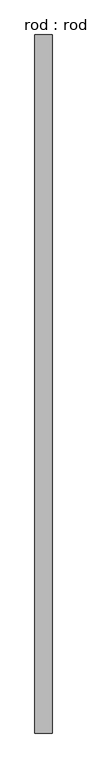
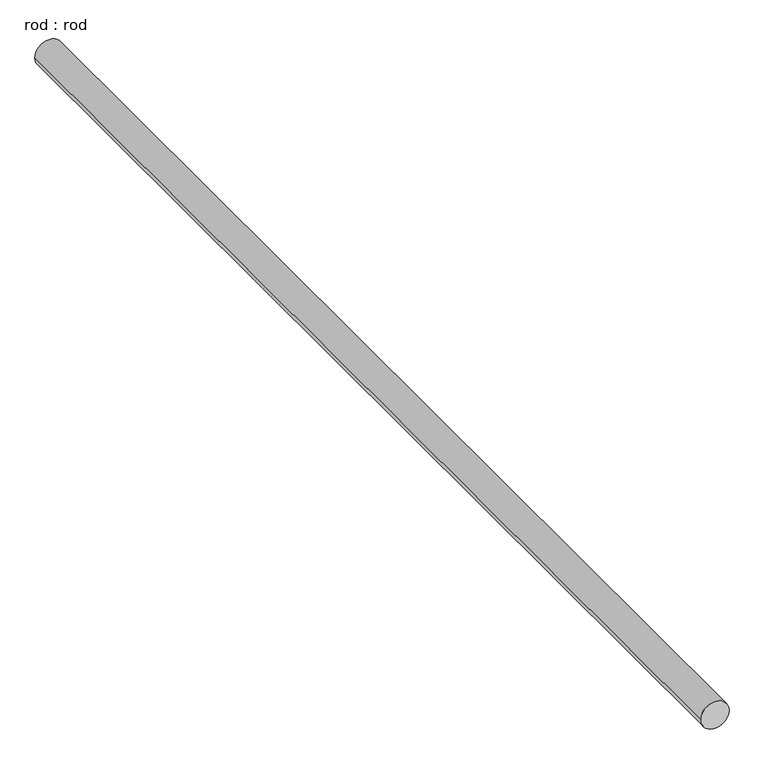
"""IFC4 building model written with IfcOpenShell, lengths in millimetres: proxy geometry, rod : rod."""

import ifcopenshell
import ifcopenshell.guid

model = None  # the IFC model being written
_history = None  # IfcOwnerHistory: only IFC2X3 demands one
_inside = {}  # id of a spatial element -> (the spatial element, [elements in it])
_under = {}  # id of a project, library or spatial element -> (it, [spatial elements below it])
_declared = {}  # id of a project -> (the project, [libraries it declares])
_typed = {}  # id of a type object -> (the type object, [elements of that type])
_made_of = {}  # id of a material, layer set ... -> (it, [elements and type objects made of it])


def new_model(schema):
    """Start an empty IFC model of exactly this schema.

    Asked for "IFC4X3", IfcOpenShell would pick the latest addendum, in which some entities
    have other attributes; the version numbers below select the first issue.
    IFC2X3 requires an IfcOwnerHistory on every rooted entity: one is made here for all.
    """
    global model, _history
    if schema == "IFC4X3":
        model = ifcopenshell.file(schema_version=(4, 3, 0, 0))
    else:
        model = ifcopenshell.file(schema=schema)
    _inside.clear()
    _under.clear()
    _declared.clear()
    _typed.clear()
    _made_of.clear()
    _history = None
    if model.schema == "IFC2X3":
        org = make("IfcOrganization", Name="unknown")
        user = make(
            "IfcPersonAndOrganization",
            ThePerson=make("IfcPerson", FamilyName="unknown"),
            TheOrganization=org,
        )
        app = make(
            "IfcApplication",
            ApplicationDeveloper=org,
            Version="unknown",
            ApplicationFullName="unknown",
            ApplicationIdentifier="unknown",
        )
        _history = make(
            "IfcOwnerHistory",
            OwningUser=user,
            OwningApplication=app,
            ChangeAction="ADDED",
            CreationDate=0,
        )
    return model


def make(cls, **values):
    """One entity of the class cls with the attributes given. An attribute that is None is left unset."""
    return model.create_entity(
        cls, **{name: value for name, value in values.items() if value is not None}
    )


def rooted(cls, **values):
    """An entity with a GlobalId (a new one), such as an element, a storey or a relation."""
    return make(cls, GlobalId=ifcopenshell.guid.new(), OwnerHistory=_history, **values)


def si_unit(unit_type, name, prefix=None):
    """IfcSIUnit, for example si_unit("LENGTHUNIT", "METRE", prefix="MILLI")."""
    return make("IfcSIUnit", UnitType=unit_type, Prefix=prefix, Name=name)


def assignment(units):
    """IfcUnitAssignment: the units of a project."""
    return None if units is None else make("IfcUnitAssignment", Units=units)


def point(xyz):
    """IfcCartesianPoint."""
    return None if xyz is None else make("IfcCartesianPoint", Coordinates=xyz)


def direction(xyz):
    """IfcDirection."""
    return None if xyz is None else make("IfcDirection", DirectionRatios=xyz)


def frame(location, z_axis=None, x_axis=None):
    """IfcAxis2Placement3D, a coordinate frame: its origin and axes. An axis left out is left unset."""
    return make(
        "IfcAxis2Placement3D",
        Location=point(location),
        Axis=direction(z_axis),
        RefDirection=direction(x_axis),
    )


def frame_2d(location, x_axis=None):
    """IfcAxis2Placement2D, a coordinate frame in the plane: its origin and x axis."""
    return make(
        "IfcAxis2Placement2D", Location=point(location), RefDirection=direction(x_axis)
    )


def origin():
    """The frame at (0, 0, 0) with its axes left unset."""
    return frame((0.0, 0.0, 0.0))


def place(relative_to, where):
    """IfcLocalPlacement: puts the frame where relative to a parent placement (None: the world)."""
    return make(
        "IfcLocalPlacement", PlacementRelTo=relative_to, RelativePlacement=where
    )


def context(
    kind, dimensions, precision=None, world=None, true_north=None, identifier=None
):
    """IfcGeometricRepresentationContext, for example the 3D "Model" context."""
    return make(
        "IfcGeometricRepresentationContext",
        ContextIdentifier=identifier,
        ContextType=kind,
        CoordinateSpaceDimension=dimensions,
        Precision=precision,
        WorldCoordinateSystem=world,
        TrueNorth=true_north,
    )


def project(units=None, contexts=None):
    """IfcProject with its units and contexts."""
    return rooted(
        "IfcProject",
        Name="project",
        RepresentationContexts=contexts,
        UnitsInContext=assignment(units),
    )


def spatial(cls, under=None, at=None, **own):
    """A site, building, storey or space (cls), placed at a placement, below another one or the project."""
    s = rooted(cls, ObjectPlacement=at, **own)
    if under is not None:
        _under.setdefault(under.id(), (under, []))[1].append(s)
    return s


def circle_curve(where, radius):
    """IfcCircle in the frame where."""
    return make("IfcCircle", Position=where, Radius=radius)


def trimmed(basis, trim1, trim2, sense, master):
    """IfcTrimmedCurve: the piece of a basis curve between two trims."""
    return make(
        "IfcTrimmedCurve",
        BasisCurve=basis,
        Trim1=trim1,
        Trim2=trim2,
        SenseAgreement=sense,
        MasterRepresentation=master,
    )


def segment(curve, same_sense, transition):
    """IfcCompositeCurveSegment."""
    return make(
        "IfcCompositeCurveSegment",
        Transition=transition,
        SameSense=same_sense,
        ParentCurve=curve,
    )


def composite_curve(segments, self_intersect=None):
    """IfcCompositeCurve: segments joined end to end."""
    return make("IfcCompositeCurve", Segments=segments, SelfIntersect=self_intersect)


def outline(outer, holes=None, kind="AREA"):
    """IfcArbitraryClosedProfileDef: a profile drawn as a closed curve; with holes, ...WithVoids."""
    if holes is None:
        return make("IfcArbitraryClosedProfileDef", ProfileType=kind, OuterCurve=outer)
    return make(
        "IfcArbitraryProfileDefWithVoids",
        ProfileType=kind,
        OuterCurve=outer,
        InnerCurves=holes,
    )


def extrude(swept, where, along, depth):
    """IfcExtrudedAreaSolid: the profile swept, set in the frame where, extruded along a direction by depth."""
    return make(
        "IfcExtrudedAreaSolid",
        SweptArea=swept,
        Position=where,
        ExtrudedDirection=direction(along),
        Depth=depth,
    )


def shape(context_of_items, identifier, shape_type, items):
    """IfcShapeRepresentation: the items that make up one representation, for example the "Body"."""
    return make(
        "IfcShapeRepresentation",
        ContextOfItems=context_of_items,
        RepresentationIdentifier=identifier,
        RepresentationType=shape_type,
        Items=items,
    )


def source(mapping_origin, context_of_items, identifier, shape_type, items):
    """IfcRepresentationMap: a shape defined once, which mapped items show again and again."""
    return make(
        "IfcRepresentationMap",
        MappingOrigin=mapping_origin,
        MappedRepresentation=shape(context_of_items, identifier, shape_type, items),
    )


def transform(
    local_origin,
    x_axis=None,
    y_axis=None,
    z_axis=None,
    scale=None,
    scale2=None,
    scale3=None,
    uniform=True,
):
    """IfcCartesianTransformationOperator3D, or its non-uniform kind. x_axis, y_axis, z_axis: its Axis1, 2, 3."""
    if uniform:
        return make(
            "IfcCartesianTransformationOperator3D",
            Axis1=direction(x_axis),
            Axis2=direction(y_axis),
            LocalOrigin=point(local_origin),
            Scale=scale,
            Axis3=direction(z_axis),
        )
    return make(
        "IfcCartesianTransformationOperator3DnonUniform",
        Axis1=direction(x_axis),
        Axis2=direction(y_axis),
        LocalOrigin=point(local_origin),
        Scale=scale,
        Axis3=direction(z_axis),
        Scale2=scale2,
        Scale3=scale3,
    )


def mapped(mapping_source, mapping_target):
    """IfcMappedItem: shows the shape of a source again, moved by a transform."""
    return make(
        "IfcMappedItem", MappingSource=mapping_source, MappingTarget=mapping_target
    )


def made_of(thing, what):
    """Note that an element or type object is made of a material, layer set ...; save() writes the relation."""
    if what is not None:
        _made_of.setdefault(what.id(), (what, []))[1].append(thing)
    return thing


def element(
    cls,
    number,
    at=None,
    inside=None,
    cuts=None,
    type_object=None,
    material=None,
    context=None,
    identifier="Body",
    shape_type=None,
    held_by="IfcProductDefinitionShape",
    body=None,
    shapes=None,
    **own,
):
    """One element of the class cls, such as IfcWall. Its Tag is "e" and its number.

    at: its placement. inside: the storey or other place that contains it. cuts: it is an
    opening in that element (IfcRelVoidsElement). A single representation is given by context,
    identifier, shape_type and body (its items); several are given by shapes. held_by: the class
    of the entity that holds the representations. save() writes the other relations.
    """
    e = rooted(cls, Tag="e%d" % number, ObjectPlacement=at, **own)
    if body is not None:
        shapes = [shape(context, identifier, shape_type, body)]
    if shapes is not None:
        e.Representation = make(held_by, Representations=shapes)
    if inside is not None:
        _inside.setdefault(inside.id(), (inside, []))[1].append(e)
    if cuts is not None:
        rooted(
            "IfcRelVoidsElement", RelatingBuildingElement=cuts, RelatedOpeningElement=e
        )
    if type_object is not None:
        _typed.setdefault(type_object.id(), (type_object, []))[1].append(e)
    return made_of(e, material)


def aggregate(whole, parts):
    """IfcRelAggregates: a whole, such as a stair, and the parts it consists of."""
    return rooted("IfcRelAggregates", RelatingObject=whole, RelatedObjects=parts)


def save(model, path):
    """Write the relations noted so far, then the file.

    IfcRelAggregates (storeys below a building ...), IfcRelContainedInSpatialStructure (elements
    in a storey), IfcRelDefinesByType, IfcRelAssociatesMaterial and IfcRelDeclares: one each for
    every whole, place, type object, material and project.
    """
    for whole, parts in _under.values():
        aggregate(whole, parts)
    for where, things in _inside.values():
        rooted(
            "IfcRelContainedInSpatialStructure",
            RelatedElements=things,
            RelatingStructure=where,
        )
    for kind, things in _typed.values():
        rooted("IfcRelDefinesByType", RelatedObjects=things, RelatingType=kind)
    for what, things in _made_of.values():
        rooted("IfcRelAssociatesMaterial", RelatedObjects=things, RelatingMaterial=what)
    for by, libraries in _declared.values():
        rooted("IfcRelDeclares", RelatingContext=by, RelatedDefinitions=libraries)
    model.write(path)


def rod_rod_62beb118(model_context):
    return source(origin(), model_context, "Body", "SweptSolid", [
        extrude(outline(composite_curve([segment(trimmed(circle_curve(frame_2d((0.0108462, 0.0)), 200.0), [point((0.0108462, 200.0))], [point((0.0108462, -200.0))], False, "CARTESIAN"), True, "CONTINUOUS"), segment(trimmed(circle_curve(frame_2d((0.0108462, 0.0)), 200.0), [point((0.0108462, -200.0))], [point((0.0108462, 200.0))], False, "CARTESIAN"), True, "CONTINUOUS")], self_intersect=False)), frame((0.0, -4039.1706397, 0.0), z_axis=(0.0, 1.0, 0.0), x_axis=(0.0, 0.0, 1.0)), (0.0, 0.0, 1.0), 16263.79851),
    ])


if __name__ == "__main__":
    model = new_model("IFC4")
    model_context = context("Model", 3, world=origin())
    ifc_project = project(units=[si_unit("LENGTHUNIT", "METRE", prefix="MILLI")], contexts=[model_context])
    site = spatial("IfcSite", under=ifc_project)
    building = spatial("IfcBuilding", under=site)
    placement = place(None, origin())
    rod_rod_shape = rod_rod_62beb118(model_context)
    element("IfcBuildingElementProxy", 1, Name="rod : rod", ObjectType="rod : rod", at=placement, inside=building, context=model_context, shape_type="MappedRepresentation", body=[
        mapped(rod_rod_shape, transform((0.0, 0.0, 0.0), x_axis=(1.0, 0.0, 0.0), y_axis=(0.0, 1.0, 0.0), z_axis=(0.0, 0.0, 1.0))),
    ])
    save(model, "model.ifc")

# Revit data of these elements
# Type "rod : rod"
#   Default Elevation = 0
